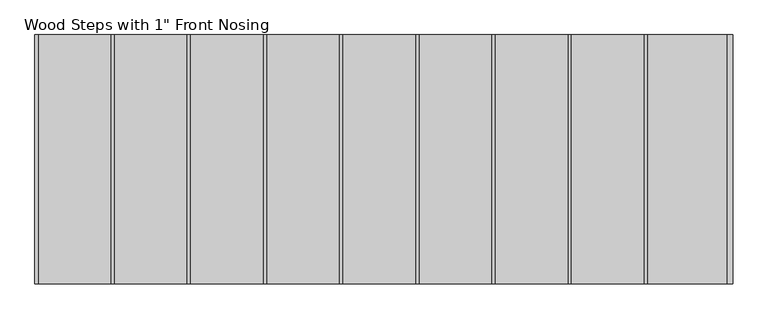
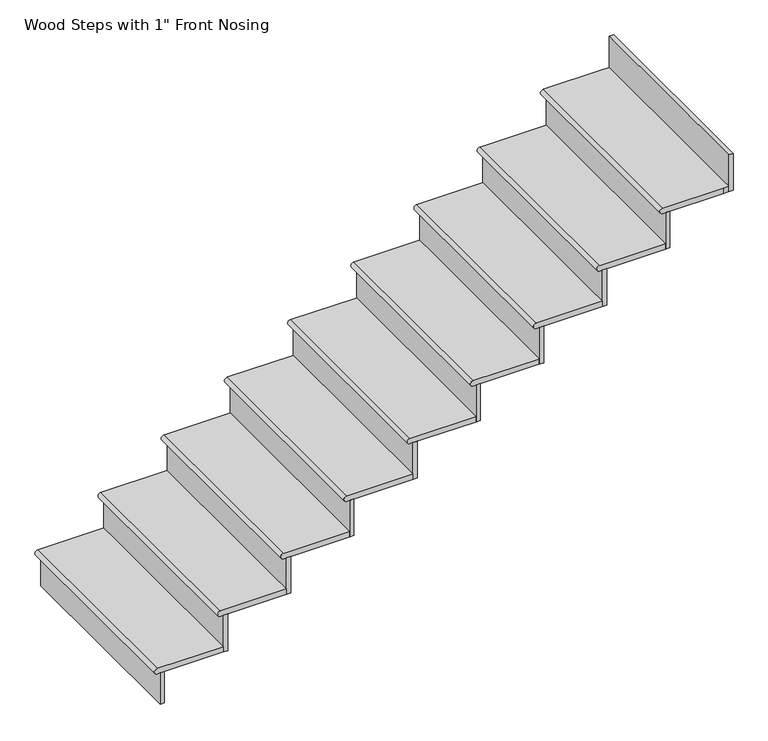
"""IFC4 building model written with IfcOpenShell, lengths in millimetres: stair flight geometry."""

from ifc_helpers import new_model, si_unit, frame, origin, place, context, project, spatial, circle_curve, faceted_brep, source, transform, mapped, element, save
from ifc_brep_helpers import plane_surface, cylinder_surface, advanced_brep


def stair_flight_bb49cb81(model_context):
    return source(origin(), model_context, "Body", "SolidModel", [
        advanced_brep(
        [(3725.1741968, -13363.3557429, 146.05), (3725.1741968, -13363.3557429, 171.45), (3725.1741968, -12448.9557429, 171.45), (3725.1741968, -12448.9557429, 146.05), (4017.2741968, -12448.9557429, 171.45), (4017.2741968, -13363.3557429, 171.45), (4017.2741968, -12448.9557429, 146.05), (4017.2741968, -13363.3557429, 146.05)],
        [
            (0, 1, circle_curve(frame((3725.1741968, -13363.3557429, 158.75), z_axis=(0.0, 1.0, 0.0), x_axis=(1.0, 0.0, 0.0)), 12.7)),
            (1, 2),
            (2, 3, circle_curve(frame((3725.1741968, -12448.9557429, 158.75), z_axis=(0.0, -1.0, 0.0), x_axis=(1.0, 0.0, 0.0)), 12.7)),
            (3, 0),
            (4, 2),
            (1, 5),
            (5, 4),
            (3, 6),
            (6, 7),
            (7, 0),
            (4, 6),
            (7, 5),
        ],
        [
            cylinder_surface(frame((3725.1741968, -13363.3557429, 158.75), z_axis=(0.0, -1.0, 0.0), x_axis=(1.0, 0.0, 0.0)), 12.7),
            plane_surface(frame((3712.4741968, -12448.9557429, 171.45), z_axis=(0.0, 0.0, 1.0), x_axis=(-1.0, 0.0, 0.0))),
            plane_surface(frame((3712.4741968, -12448.9557429, 146.05), z_axis=(0.0, 0.0, -1.0), x_axis=(1.0, 0.0, 0.0))),
            plane_surface(frame((4017.2741968, -12448.9557429, 171.45), z_axis=(0.0, 1.0, 0.0), x_axis=(0.0, 0.0, -1.0))),
            plane_surface(frame((3725.1741968, -13363.3557429, 171.45), z_axis=(0.0, -1.0, 0.0), x_axis=(0.0, 0.0, -1.0))),
            plane_surface(frame((4017.2741968, -13363.3557429, 171.45), z_axis=(1.0, 0.0, 0.0), x_axis=(0.0, 0.0, -1.0))),
        ],
        [
            (0, [[1, 2, 3, 4]]),
            (1, [[5, -2, 6, 7]]),
            (2, [[8, 9, 10, -4]]),
            (3, [[-5, 11, -8, -3]]),
            (4, [[-6, -1, -10, 12]]),
            (5, [[-7, -12, -9, -11]]),
        ],
    ),
        faceted_brep([(3737.8741968, -13363.3557429, 146.05), (3737.8741968, -13363.3557429, 0.0), (3756.9241968, -13363.3557429, 0.0), (3756.9241968, -13363.3557429, 146.05), (3737.8741968, -12448.9557429, 146.05), (3756.9241968, -12448.9557429, 146.05), (3756.9241968, -12448.9557429, 0.0), (3737.8741968, -12448.9557429, 0.0)], [[[0, 1, 2, 3]], [[4, 5, 6, 7]], [[1, 0, 4, 7]], [[2, 1, 7, 6]], [[3, 2, 6, 5]], [[0, 3, 5, 4]]]),
        faceted_brep([(4017.2741968, -13363.3557429, 317.5), (4017.2741968, -13363.3557429, 146.05), (4036.3241968, -13363.3557429, 146.05), (4036.3241968, -13363.3557429, 317.5), (4017.2741968, -12448.9557429, 317.5), (4036.3241968, -12448.9557429, 317.5), (4036.3241968, -12448.9557429, 146.05), (4017.2741968, -12448.9557429, 146.05)], [[[0, 1, 2, 3]], [[4, 5, 6, 7]], [[1, 0, 4, 7]], [[2, 1, 7, 6]], [[3, 2, 6, 5]], [[0, 3, 5, 4]]]),
        advanced_brep(
        [(4296.6741968, -12448.9557429, 342.9), (4004.5741968, -12448.9557429, 342.9), (4004.5741968, -13363.3557429, 342.9), (4296.6741968, -13363.3557429, 342.9), (4004.5741968, -12448.9557429, 317.5), (4296.6741968, -12448.9557429, 317.5), (4296.6741968, -13363.3557429, 317.5), (4004.5741968, -13363.3557429, 317.5)],
        [
            (0, 1),
            (1, 2),
            (2, 3),
            (3, 0),
            (4, 5),
            (5, 6),
            (6, 7),
            (7, 4),
            (0, 5),
            (4, 1, circle_curve(frame((4004.5741968, -12448.9557429, 330.2), z_axis=(0.0, 1.0, 0.0), x_axis=(1.0, 0.0, 0.0)), 12.7)),
            (2, 7, circle_curve(frame((4004.5741968, -13363.3557429, 330.2), z_axis=(0.0, -1.0, 0.0), x_axis=(1.0, 0.0, 0.0)), 12.7)),
            (6, 3),
        ],
        [
            plane_surface(frame((3712.4741968, -12448.9557429, 342.9), z_axis=(0.0, 0.0, 1.0), x_axis=(-1.0, 0.0, 0.0))),
            plane_surface(frame((3712.4741968, -12448.9557429, 317.5), z_axis=(0.0, 0.0, -1.0), x_axis=(1.0, 0.0, 0.0))),
            plane_surface(frame((4296.6741968, -12448.9557429, 342.9), z_axis=(0.0, 1.0, 0.0), x_axis=(0.0, 0.0, -1.0))),
            plane_surface(frame((4004.5741968, -13363.3557429, 342.9), z_axis=(0.0, -1.0, 0.0), x_axis=(0.0, 0.0, -1.0))),
            plane_surface(frame((4296.6741968, -13363.3557429, 342.9), z_axis=(1.0, 0.0, 0.0), x_axis=(0.0, 0.0, -1.0))),
            cylinder_surface(frame((4004.5741968, -13363.3557429, 330.2), z_axis=(0.0, -1.0, 0.0), x_axis=(1.0, 0.0, 0.0)), 12.7),
        ],
        [
            (0, [[1, 2, 3, 4]]),
            (1, [[5, 6, 7, 8]]),
            (2, [[-1, 9, -5, 10]]),
            (3, [[-3, 11, -7, 12]]),
            (4, [[-4, -12, -6, -9]]),
            (5, [[-11, -2, -10, -8]]),
        ],
    ),
        faceted_brep([(4296.6741968, -13363.3557429, 488.95), (4296.6741968, -13363.3557429, 317.5), (4315.7241968, -13363.3557429, 317.5), (4315.7241968, -13363.3557429, 488.95), (4296.6741968, -12448.9557429, 488.95), (4315.7241968, -12448.9557429, 488.95), (4315.7241968, -12448.9557429, 317.5), (4296.6741968, -12448.9557429, 317.5)], [[[0, 1, 2, 3]], [[4, 5, 6, 7]], [[1, 0, 4, 7]], [[2, 1, 7, 6]], [[3, 2, 6, 5]], [[0, 3, 5, 4]]]),
        advanced_brep(
        [(4576.0741968, -12448.9557429, 514.35), (4283.9741968, -12448.9557429, 514.35), (4283.9741968, -13363.3557429, 514.35), (4576.0741968, -13363.3557429, 514.35), (4283.9741968, -12448.9557429, 488.95), (4576.0741968, -12448.9557429, 488.95), (4576.0741968, -13363.3557429, 488.95), (4283.9741968, -13363.3557429, 488.95)],
        [
            (0, 1),
            (1, 2),
            (2, 3),
            (3, 0),
            (4, 5),
            (5, 6),
            (6, 7),
            (7, 4),
            (0, 5),
            (4, 1, circle_curve(frame((4283.9741968, -12448.9557429, 501.65), z_axis=(0.0, 1.0, 0.0), x_axis=(1.0, 0.0, 0.0)), 12.7)),
            (2, 7, circle_curve(frame((4283.9741968, -13363.3557429, 501.65), z_axis=(0.0, -1.0, 0.0), x_axis=(1.0, 0.0, 0.0)), 12.7)),
            (6, 3),
        ],
        [
            plane_surface(frame((3991.8741968, -12448.9557429, 514.35), z_axis=(0.0, 0.0, 1.0), x_axis=(-1.0, 0.0, 0.0))),
            plane_surface(frame((3991.8741968, -12448.9557429, 488.95), z_axis=(0.0, 0.0, -1.0), x_axis=(1.0, 0.0, 0.0))),
            plane_surface(frame((4576.0741968, -12448.9557429, 514.35), z_axis=(0.0, 1.0, 0.0), x_axis=(0.0, 0.0, -1.0))),
            plane_surface(frame((4283.9741968, -13363.3557429, 514.35), z_axis=(0.0, -1.0, 0.0), x_axis=(0.0, 0.0, -1.0))),
            plane_surface(frame((4576.0741968, -13363.3557429, 514.35), z_axis=(1.0, 0.0, 0.0), x_axis=(0.0, 0.0, -1.0))),
            cylinder_surface(frame((4283.9741968, -13363.3557429, 501.65), z_axis=(0.0, -1.0, 0.0), x_axis=(1.0, 0.0, 0.0)), 12.7),
        ],
        [
            (0, [[1, 2, 3, 4]]),
            (1, [[5, 6, 7, 8]]),
            (2, [[-1, 9, -5, 10]]),
            (3, [[-3, 11, -7, 12]]),
            (4, [[-4, -12, -6, -9]]),
            (5, [[-11, -2, -10, -8]]),
        ],
    ),
        faceted_brep([(4576.0741968, -13363.3557429, 660.4), (4576.0741968, -13363.3557429, 488.95), (4595.1241968, -13363.3557429, 488.95), (4595.1241968, -13363.3557429, 660.4), (4576.0741968, -12448.9557429, 660.4), (4595.1241968, -12448.9557429, 660.4), (4595.1241968, -12448.9557429, 488.95), (4576.0741968, -12448.9557429, 488.95)], [[[0, 1, 2, 3]], [[4, 5, 6, 7]], [[1, 0, 4, 7]], [[2, 1, 7, 6]], [[3, 2, 6, 5]], [[0, 3, 5, 4]]]),
        advanced_brep(
        [(4855.4741968, -12448.9557429, 685.8), (4563.3741968, -12448.9557429, 685.8), (4563.3741968, -13363.3557429, 685.8), (4855.4741968, -13363.3557429, 685.8), (4563.3741968, -12448.9557429, 660.4), (4855.4741968, -12448.9557429, 660.4), (4855.4741968, -13363.3557429, 660.4), (4563.3741968, -13363.3557429, 660.4)],
        [
            (0, 1),
            (1, 2),
            (2, 3),
            (3, 0),
            (4, 5),
            (5, 6),
            (6, 7),
            (7, 4),
            (0, 5),
            (4, 1, circle_curve(frame((4563.3741968, -12448.9557429, 673.1), z_axis=(0.0, 1.0, 0.0), x_axis=(1.0, 0.0, 0.0)), 12.7)),
            (2, 7, circle_curve(frame((4563.3741968, -13363.3557429, 673.1), z_axis=(0.0, -1.0, 0.0), x_axis=(1.0, 0.0, 0.0)), 12.7)),
            (6, 3),
        ],
        [
            plane_surface(frame((4271.2741968, -12448.9557429, 685.8), z_axis=(0.0, 0.0, 1.0), x_axis=(-1.0, 0.0, 0.0))),
            plane_surface(frame((4271.2741968, -12448.9557429, 660.4), z_axis=(0.0, 0.0, -1.0), x_axis=(1.0, 0.0, 0.0))),
            plane_surface(frame((4855.4741968, -12448.9557429, 685.8), z_axis=(0.0, 1.0, 0.0), x_axis=(0.0, 0.0, -1.0))),
            plane_surface(frame((4563.3741968, -13363.3557429, 685.8), z_axis=(0.0, -1.0, 0.0), x_axis=(0.0, 0.0, -1.0))),
            plane_surface(frame((4855.4741968, -13363.3557429, 685.8), z_axis=(1.0, 0.0, 0.0), x_axis=(0.0, 0.0, -1.0))),
            cylinder_surface(frame((4563.3741968, -13363.3557429, 673.1), z_axis=(0.0, -1.0, 0.0), x_axis=(1.0, 0.0, 0.0)), 12.7),
        ],
        [
            (0, [[1, 2, 3, 4]]),
            (1, [[5, 6, 7, 8]]),
            (2, [[-1, 9, -5, 10]]),
            (3, [[-3, 11, -7, 12]]),
            (4, [[-4, -12, -6, -9]]),
            (5, [[-11, -2, -10, -8]]),
        ],
    ),
        faceted_brep([(4855.4741968, -13363.3557429, 831.85), (4855.4741968, -13363.3557429, 660.4), (4874.5241968, -13363.3557429, 660.4), (4874.5241968, -13363.3557429, 831.85), (4855.4741968, -12448.9557429, 831.85), (4874.5241968, -12448.9557429, 831.85), (4874.5241968, -12448.9557429, 660.4), (4855.4741968, -12448.9557429, 660.4)], [[[0, 1, 2, 3]], [[4, 5, 6, 7]], [[1, 0, 4, 7]], [[2, 1, 7, 6]], [[3, 2, 6, 5]], [[0, 3, 5, 4]]]),
        advanced_brep(
        [(5134.8741968, -12448.9557429, 857.25), (4842.7741968, -12448.9557429, 857.25), (4842.7741968, -13363.3557429, 857.25), (5134.8741968, -13363.3557429, 857.25), (4842.7741968, -12448.9557429, 831.85), (5134.8741968, -12448.9557429, 831.85), (5134.8741968, -13363.3557429, 831.85), (4842.7741968, -13363.3557429, 831.85)],
        [
            (0, 1),
            (1, 2),
            (2, 3),
            (3, 0),
            (4, 5),
            (5, 6),
            (6, 7),
            (7, 4),
            (0, 5),
            (4, 1, circle_curve(frame((4842.7741968, -12448.9557429, 844.55), z_axis=(0.0, 1.0, 0.0), x_axis=(1.0, 0.0, 0.0)), 12.7)),
            (2, 7, circle_curve(frame((4842.7741968, -13363.3557429, 844.55), z_axis=(0.0, -1.0, 0.0), x_axis=(1.0, 0.0, 0.0)), 12.7)),
            (6, 3),
        ],
        [
            plane_surface(frame((4550.6741968, -12448.9557429, 857.25), z_axis=(0.0, 0.0, 1.0), x_axis=(-1.0, 0.0, 0.0))),
            plane_surface(frame((4550.6741968, -12448.9557429, 831.85), z_axis=(0.0, 0.0, -1.0), x_axis=(1.0, 0.0, 0.0))),
            plane_surface(frame((5134.8741968, -12448.9557429, 857.25), z_axis=(0.0, 1.0, 0.0), x_axis=(0.0, 0.0, -1.0))),
            plane_surface(frame((4842.7741968, -13363.3557429, 857.25), z_axis=(0.0, -1.0, 0.0), x_axis=(0.0, 0.0, -1.0))),
            plane_surface(frame((5134.8741968, -13363.3557429, 857.25), z_axis=(1.0, 0.0, 0.0), x_axis=(0.0, 0.0, -1.0))),
            cylinder_surface(frame((4842.7741968, -13363.3557429, 844.55), z_axis=(0.0, -1.0, 0.0), x_axis=(1.0, 0.0, 0.0)), 12.7),
        ],
        [
            (0, [[1, 2, 3, 4]]),
            (1, [[5, 6, 7, 8]]),
            (2, [[-1, 9, -5, 10]]),
            (3, [[-3, 11, -7, 12]]),
            (4, [[-4, -12, -6, -9]]),
            (5, [[-11, -2, -10, -8]]),
        ],
    ),
        faceted_brep([(5134.8741968, -13363.3557429, 1003.3), (5134.8741968, -13363.3557429, 831.85), (5153.9241968, -13363.3557429, 831.85), (5153.9241968, -13363.3557429, 1003.3), (5134.8741968, -12448.9557429, 1003.3), (5153.9241968, -12448.9557429, 1003.3), (5153.9241968, -12448.9557429, 831.85), (5134.8741968, -12448.9557429, 831.85)], [[[0, 1, 2, 3]], [[4, 5, 6, 7]], [[1, 0, 4, 7]], [[2, 1, 7, 6]], [[3, 2, 6, 5]], [[0, 3, 5, 4]]]),
        advanced_brep(
        [(5414.2741968, -12448.9557429, 1028.7), (5122.1741968, -12448.9557429, 1028.7), (5122.1741968, -13363.3557429, 1028.7), (5414.2741968, -13363.3557429, 1028.7), (5122.1741968, -12448.9557429, 1003.3), (5414.2741968, -12448.9557429, 1003.3), (5414.2741968, -13363.3557429, 1003.3), (5122.1741968, -13363.3557429, 1003.3)],
        [
            (0, 1),
            (1, 2),
            (2, 3),
            (3, 0),
            (4, 5),
            (5, 6),
            (6, 7),
            (7, 4),
            (0, 5),
            (4, 1, circle_curve(frame((5122.1741968, -12448.9557429, 1016.0), z_axis=(0.0, 1.0, 0.0), x_axis=(1.0, 0.0, 0.0)), 12.7)),
            (2, 7, circle_curve(frame((5122.1741968, -13363.3557429, 1016.0), z_axis=(0.0, -1.0, 0.0), x_axis=(1.0, 0.0, 0.0)), 12.7)),
            (6, 3),
        ],
        [
            plane_surface(frame((4830.0741968, -12448.9557429, 1028.7), z_axis=(0.0, 0.0, 1.0), x_axis=(-1.0, 0.0, 0.0))),
            plane_surface(frame((4830.0741968, -12448.9557429, 1003.3), z_axis=(0.0, 0.0, -1.0), x_axis=(1.0, 0.0, 0.0))),
            plane_surface(frame((5414.2741968, -12448.9557429, 1028.7), z_axis=(0.0, 1.0, 0.0), x_axis=(0.0, 0.0, -1.0))),
            plane_surface(frame((5122.1741968, -13363.3557429, 1028.7), z_axis=(0.0, -1.0, 0.0), x_axis=(0.0, 0.0, -1.0))),
            plane_surface(frame((5414.2741968, -13363.3557429, 1028.7), z_axis=(1.0, 0.0, 0.0), x_axis=(0.0, 0.0, -1.0))),
            cylinder_surface(frame((5122.1741968, -13363.3557429, 1016.0), z_axis=(0.0, -1.0, 0.0), x_axis=(1.0, 0.0, 0.0)), 12.7),
        ],
        [
            (0, [[1, 2, 3, 4]]),
            (1, [[5, 6, 7, 8]]),
            (2, [[-1, 9, -5, 10]]),
            (3, [[-3, 11, -7, 12]]),
            (4, [[-4, -12, -6, -9]]),
            (5, [[-11, -2, -10, -8]]),
        ],
    ),
        faceted_brep([(5414.2741968, -13363.3557429, 1174.75), (5414.2741968, -13363.3557429, 1003.3), (5433.3241968, -13363.3557429, 1003.3), (5433.3241968, -13363.3557429, 1174.75), (5414.2741968, -12448.9557429, 1174.75), (5433.3241968, -12448.9557429, 1174.75), (5433.3241968, -12448.9557429, 1003.3), (5414.2741968, -12448.9557429, 1003.3)], [[[0, 1, 2, 3]], [[4, 5, 6, 7]], [[1, 0, 4, 7]], [[2, 1, 7, 6]], [[3, 2, 6, 5]], [[0, 3, 5, 4]]]),
        advanced_brep(
        [(5693.6741968, -12448.9557429, 1200.15), (5401.5741968, -12448.9557429, 1200.15), (5401.5741968, -13363.3557429, 1200.15), (5693.6741968, -13363.3557429, 1200.15), (5401.5741968, -12448.9557429, 1174.75), (5693.6741968, -12448.9557429, 1174.75), (5693.6741968, -13363.3557429, 1174.75), (5401.5741968, -13363.3557429, 1174.75)],
        [
            (0, 1),
            (1, 2),
            (2, 3),
            (3, 0),
            (4, 5),
            (5, 6),
            (6, 7),
            (7, 4),
            (0, 5),
            (4, 1, circle_curve(frame((5401.5741968, -12448.9557429, 1187.45), z_axis=(0.0, 1.0, 0.0), x_axis=(1.0, 0.0, 0.0)), 12.7)),
            (2, 7, circle_curve(frame((5401.5741968, -13363.3557429, 1187.45), z_axis=(0.0, -1.0, 0.0), x_axis=(1.0, 0.0, 0.0)), 12.7)),
            (6, 3),
        ],
        [
            plane_surface(frame((5109.4741968, -12448.9557429, 1200.15), z_axis=(0.0, 0.0, 1.0), x_axis=(-1.0, 0.0, 0.0))),
            plane_surface(frame((5109.4741968, -12448.9557429, 1174.75), z_axis=(0.0, 0.0, -1.0), x_axis=(1.0, 0.0, 0.0))),
            plane_surface(frame((5693.6741968, -12448.9557429, 1200.15), z_axis=(0.0, 1.0, 0.0), x_axis=(0.0, 0.0, -1.0))),
            plane_surface(frame((5401.5741968, -13363.3557429, 1200.15), z_axis=(0.0, -1.0, 0.0), x_axis=(0.0, 0.0, -1.0))),
            plane_surface(frame((5693.6741968, -13363.3557429, 1200.15), z_axis=(1.0, 0.0, 0.0), x_axis=(0.0, 0.0, -1.0))),
            cylinder_surface(frame((5401.5741968, -13363.3557429, 1187.45), z_axis=(0.0, -1.0, 0.0), x_axis=(1.0, 0.0, 0.0)), 12.7),
        ],
        [
            (0, [[1, 2, 3, 4]]),
            (1, [[5, 6, 7, 8]]),
            (2, [[-1, 9, -5, 10]]),
            (3, [[-3, 11, -7, 12]]),
            (4, [[-4, -12, -6, -9]]),
            (5, [[-11, -2, -10, -8]]),
        ],
    ),
        faceted_brep([(5693.6741968, -13363.3557429, 1346.2), (5693.6741968, -13363.3557429, 1174.75), (5712.7241968, -13363.3557429, 1174.75), (5712.7241968, -13363.3557429, 1346.2), (5693.6741968, -12448.9557429, 1346.2), (5712.7241968, -12448.9557429, 1346.2), (5712.7241968, -12448.9557429, 1174.75), (5693.6741968, -12448.9557429, 1174.75)], [[[0, 1, 2, 3]], [[4, 5, 6, 7]], [[1, 0, 4, 7]], [[2, 1, 7, 6]], [[3, 2, 6, 5]], [[0, 3, 5, 4]]]),
        advanced_brep(
        [(5973.0741968, -12448.9557429, 1371.6), (5680.9741968, -12448.9557429, 1371.6), (5680.9741968, -13363.3557429, 1371.6), (5973.0741968, -13363.3557429, 1371.6), (5680.9741968, -12448.9557429, 1346.2), (5973.0741968, -12448.9557429, 1346.2), (5973.0741968, -13363.3557429, 1346.2), (5680.9741968, -13363.3557429, 1346.2)],
        [
            (0, 1),
            (1, 2),
            (2, 3),
            (3, 0),
            (4, 5),
            (5, 6),
            (6, 7),
            (7, 4),
            (0, 5),
            (4, 1, circle_curve(frame((5680.9741968, -12448.9557429, 1358.9), z_axis=(0.0, 1.0, 0.0), x_axis=(1.0, 0.0, 0.0)), 12.7)),
            (2, 7, circle_curve(frame((5680.9741968, -13363.3557429, 1358.9), z_axis=(0.0, -1.0, 0.0), x_axis=(1.0, 0.0, 0.0)), 12.7)),
            (6, 3),
        ],
        [
            plane_surface(frame((5388.8741968, -12448.9557429, 1371.6), z_axis=(0.0, 0.0, 1.0), x_axis=(-1.0, 0.0, 0.0))),
            plane_surface(frame((5388.8741968, -12448.9557429, 1346.2), z_axis=(0.0, 0.0, -1.0), x_axis=(1.0, 0.0, 0.0))),
            plane_surface(frame((5973.0741968, -12448.9557429, 1371.6), z_axis=(0.0, 1.0, 0.0), x_axis=(0.0, 0.0, -1.0))),
            plane_surface(frame((5680.9741968, -13363.3557429, 1371.6), z_axis=(0.0, -1.0, 0.0), x_axis=(0.0, 0.0, -1.0))),
            plane_surface(frame((5973.0741968, -13363.3557429, 1371.6), z_axis=(1.0, 0.0, 0.0), x_axis=(0.0, 0.0, -1.0))),
            cylinder_surface(frame((5680.9741968, -13363.3557429, 1358.9), z_axis=(0.0, -1.0, 0.0), x_axis=(1.0, 0.0, 0.0)), 12.7),
        ],
        [
            (0, [[1, 2, 3, 4]]),
            (1, [[5, 6, 7, 8]]),
            (2, [[-1, 9, -5, 10]]),
            (3, [[-3, 11, -7, 12]]),
            (4, [[-4, -12, -6, -9]]),
            (5, [[-11, -2, -10, -8]]),
        ],
    ),
        faceted_brep([(6252.4741968, -13363.3557429, 1689.1), (6252.4741968, -13363.3557429, 1517.65), (6271.5241968, -13363.3557429, 1517.65), (6271.5241968, -13363.3557429, 1689.1), (6252.4741968, -12448.9557429, 1689.1), (6271.5241968, -12448.9557429, 1689.1), (6271.5241968, -12448.9557429, 1517.65), (6252.4741968, -12448.9557429, 1517.65)], [[[0, 1, 2, 3]], [[4, 5, 6, 7]], [[1, 0, 4, 7]], [[2, 1, 7, 6]], [[3, 2, 6, 5]], [[0, 3, 5, 4]]]),
        faceted_brep([(5973.0741968, -13363.3557429, 1517.65), (5973.0741968, -13363.3557429, 1346.2), (5992.1241968, -13363.3557429, 1346.2), (5992.1241968, -13363.3557429, 1517.65), (5973.0741968, -12448.9557429, 1517.65), (5992.1241968, -12448.9557429, 1517.65), (5992.1241968, -12448.9557429, 1346.2), (5973.0741968, -12448.9557429, 1346.2)], [[[0, 1, 2, 3]], [[4, 5, 6, 7]], [[1, 0, 4, 7]], [[2, 1, 7, 6]], [[3, 2, 6, 5]], [[0, 3, 5, 4]]]),
        advanced_brep(
        [(6252.4741968, -12448.9557429, 1543.05), (6227.0741968, -12448.9557429, 1543.05), (5960.3741968, -12448.9557429, 1543.05), (5960.3741968, -13363.3557429, 1543.05), (6227.0741968, -13363.3557429, 1543.05), (6252.4741968, -13363.3557429, 1543.05), (6227.0741968, -12448.9557429, 1517.65), (6252.4741968, -12448.9557429, 1517.65), (6252.4741968, -13363.3557429, 1517.65), (6227.0741968, -13363.3557429, 1517.65), (5960.3741968, -13363.3557429, 1517.65), (5960.3741968, -12448.9557429, 1517.65)],
        [
            (0, 1),
            (1, 2),
            (2, 3),
            (3, 4),
            (4, 5),
            (5, 0),
            (6, 7),
            (7, 8),
            (8, 9),
            (9, 10),
            (10, 11),
            (11, 6),
            (0, 7),
            (6, 1),
            (11, 2, circle_curve(frame((5960.3741968, -12448.9557429, 1530.35), z_axis=(0.0, 1.0, 0.0), x_axis=(1.0, 0.0, 0.0)), 12.7)),
            (3, 10, circle_curve(frame((5960.3741968, -13363.3557429, 1530.35), z_axis=(0.0, -1.0, 0.0), x_axis=(1.0, 0.0, 0.0)), 12.7)),
            (9, 4),
            (8, 5),
        ],
        [
            plane_surface(frame((6227.0741968, -12448.9557429, 1543.05), z_axis=(0.0, 0.0, 1.0), x_axis=(-1.0, 0.0, 0.0))),
            plane_surface(frame((6227.0741968, -12448.9557429, 1517.65), z_axis=(0.0, 0.0, -1.0), x_axis=(1.0, 0.0, 0.0))),
            plane_surface(frame((6252.4741968, -12448.9557429, 1543.05), z_axis=(0.0, 1.0, 0.0), x_axis=(0.0, 0.0, -1.0))),
            plane_surface(frame((6227.0741968, -12448.9557429, 1543.05), z_axis=(0.0, 1.0, 0.0), x_axis=(0.0, 0.0, -1.0))),
            plane_surface(frame((5960.3741968, -13363.3557429, 1543.05), z_axis=(0.0, -1.0, 0.0), x_axis=(0.0, 0.0, -1.0))),
            plane_surface(frame((6227.0741968, -13363.3557429, 1543.05), z_axis=(0.0, -1.0, 0.0), x_axis=(0.0, 0.0, -1.0))),
            plane_surface(frame((6252.4741968, -13363.3557429, 1543.05), z_axis=(1.0, 0.0, 0.0), x_axis=(0.0, 0.0, -1.0))),
            cylinder_surface(frame((5960.3741968, -13363.3557429, 1530.35), z_axis=(0.0, -1.0, 0.0), x_axis=(1.0, 0.0, 0.0)), 12.7),
        ],
        [
            (0, [[1, 2, 3, 4, 5, 6]]),
            (1, [[7, 8, 9, 10, 11, 12]]),
            (2, [[-1, 13, -7, 14]]),
            (3, [[-2, -14, -12, 15]]),
            (4, [[-4, 16, -10, 17]]),
            (5, [[-5, -17, -9, 18]]),
            (6, [[-6, -18, -8, -13]]),
            (7, [[-16, -3, -15, -11]]),
        ],
    ),
    ])


if __name__ == "__main__":
    model = new_model("IFC4")
    model_context = context("Model", 3, world=origin())
    ifc_project = project(units=[si_unit("LENGTHUNIT", "METRE", prefix="MILLI")], contexts=[model_context])
    site = spatial("IfcSite", under=ifc_project)
    building = spatial("IfcBuilding", under=site)
    placement = place(None, origin())
    stair_flight_shape = stair_flight_bb49cb81(model_context)
    element("IfcStairFlight", 1, ObjectType="Wood Steps with 1\" Front Nosing", at=placement, inside=building, context=model_context, shape_type="MappedRepresentation", body=[
        mapped(stair_flight_shape, transform((0.0, 0.0, 0.0), x_axis=(1.0, 0.0, 0.0), y_axis=(0.0, 1.0, 0.0), z_axis=(0.0, 0.0, 1.0))),
    ])
    save(model, "model.ifc")

# Revit data of these elements
# Element 1 (IfcStairFlight, "Wood Steps with 1\" Front Nosing")
#   Materials on its faces: "Paints and Coatings", "Cherry"
# Materials
#   "Paints and Coatings": class "Paint", colour RGB 244 244 244, transparency 0, Description = "Interior finish", Cost = 0
#   "Cherry": class "Wood", colour RGB 233 182 144, transparency 0, Description = "Prunus Serotina", Cost = 0
